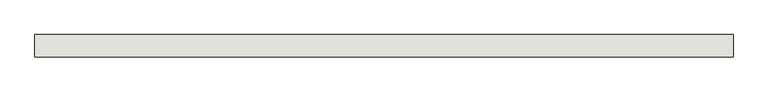
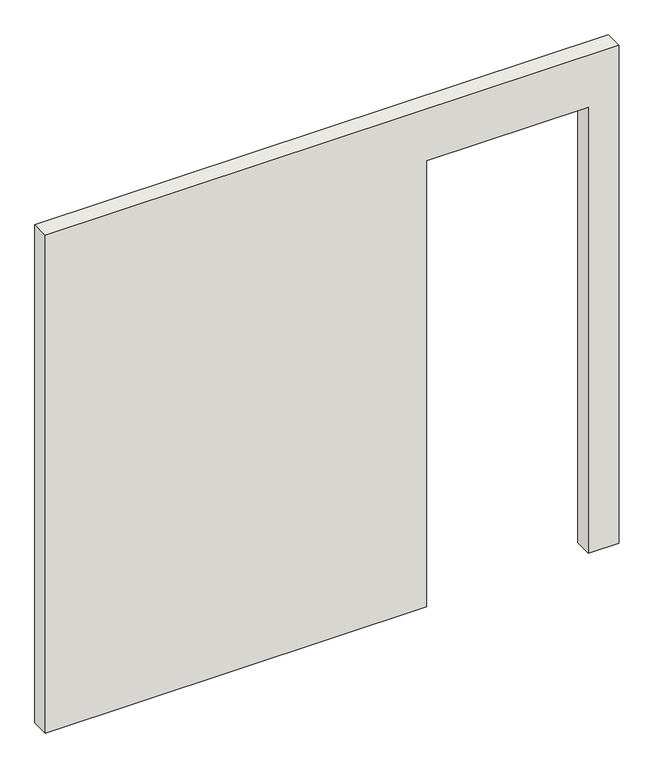
"""IFC4 building model written with IfcOpenShell, lengths in millimetres: wall geometry, 0_3d_modell."""

from ifc_helpers import new_model, si_unit, frame, origin, place, context, project, spatial, polyline, outline, extrude, source, transform, mapped, element, save


def wall_f1e99909(model_context):
    return source(origin(), model_context, "Body", "SweptSolid", [
        extrude(outline(polyline([(2580.0, 2972.9900821), (0.0, 2972.9900821), (0.0, 3139.9364642), (2880.0, 3139.9364642), (2880.0, 0.0), (0.0, 0.0), (0.0, 2087.9900821), (2580.0, 2087.9900821), (2580.0, 2972.9900821)])), frame((0.0, 0.0, 0.0), z_axis=(0.0, 1.0, 0.0), x_axis=(0.0, 0.0, 1.0)), (0.0, 0.0, 1.0), 100.0),
    ])


if __name__ == "__main__":
    model = new_model("IFC4")
    model_context = context("Model", 3, world=origin())
    ifc_project = project(units=[si_unit("LENGTHUNIT", "METRE", prefix="MILLI")], contexts=[model_context])
    site = spatial("IfcSite", under=ifc_project)
    building = spatial("IfcBuilding", under=site)
    placement = place(None, origin())
    wall_shape = wall_f1e99909(model_context)
    element("IfcWall", 1, ObjectType="0_3d_modell", at=placement, inside=building, context=model_context, shape_type="MappedRepresentation", body=[
        mapped(wall_shape, transform((0.0, 0.0, 0.0), x_axis=(1.0, 0.0, 0.0), y_axis=(0.0, 1.0, 0.0), z_axis=(0.0, 0.0, 1.0))),
    ])
    save(model, "model.ifc")

# Revit data of these elements
# Element 1 (IfcWall, "0_3d_modell")
#   Materials on its faces: "material wardrobe b 1"
# Materials
#   "material wardrobe b 1": class "Unassigned", colour RGB 128 128 128, transparency 0
